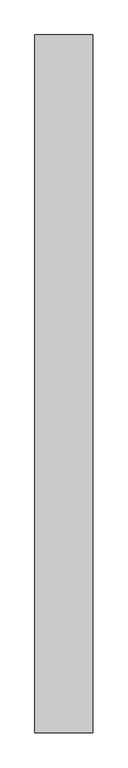
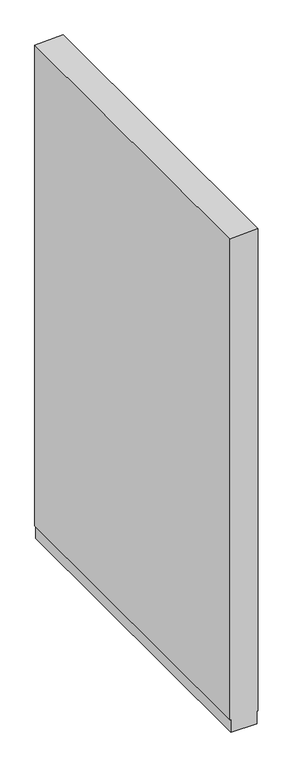
"""IFC4 building model written with IfcOpenShell, lengths in millimetres: proxy geometry, Generic Models 7:Generic Models 1:5:Generic Models 1:5 : Generic Models 7:Generic Models 1:337419:33 : Generic Models 7:Generic Models 1:5:Generic Models 1:5 : Generic Models 7:Generic Models 1:337419:311462."""

from ifc_helpers import new_model, si_unit, frame, origin, place, context, project, spatial, polyline, outline, extrude, source, transform, mapped, element, save


def generic_models_b9c952d6(model_context):
    return source(origin(), model_context, "Body", "SweptSolid", [
        extrude(outline(polyline([(103.1875, 560567.2742239), (3729.5005208, 560567.2742239), (3721.1661458, 560367.2492239), (103.1875, 560367.2492239), (103.1875, 560373.5992239), (7.9375, 560373.5992239), (7.9375, 560560.9242239), (103.1875, 560560.9242239), (103.1875, 560567.2742239)])), frame((0.0, -545590.1663841, 0.0), z_axis=(0.0, 1.0, 0.0), x_axis=(0.0, 0.0, 1.0)), (0.0, 0.0, 1.0), 2406.65),
    ])


if __name__ == "__main__":
    model = new_model("IFC4")
    model_context = context("Model", 3, world=origin())
    ifc_project = project(units=[si_unit("LENGTHUNIT", "METRE", prefix="MILLI")], contexts=[model_context])
    site = spatial("IfcSite", under=ifc_project)
    building = spatial("IfcBuilding", under=site)
    placement = place(None, origin())
    generic_models_shape = generic_models_b9c952d6(model_context)
    element("IfcBuildingElementProxy", 1, Name="Generic Models 7:Generic Models 1:5:Generic Models 1:5 : Generic Models 7:Generic Models 1:337419:33 : Generic Models 7:Generic Models 1:5:Generic Models 1:5 : Generic Models 7:Generic Models 1:337419:311462", ObjectType="Generic Models 7:Generic Models 1:5:Generic Models 1:5 : Generic Models 7:Generic Models 1:337419:33 : Generic Models 7:Generic Models 1:5:Generic Models 1:5 : Generic Models 7:Generic Models 1:337419:311462", at=placement, inside=building, context=model_context, shape_type="MappedRepresentation", body=[
        mapped(generic_models_shape, transform((0.0, 0.0, 0.0), x_axis=(1.0, 0.0, 0.0), y_axis=(0.0, 1.0, 0.0), z_axis=(0.0, 0.0, 1.0))),
    ])
    save(model, "model.ifc")

# Revit data of these elements
# Type "Generic Models 7:Generic Models 1:5:Generic Models 1:5 : Generic Models 7:Generic Models 1:337419:33 : Generic Models 7:Generic Models 1:5:Generic Models 1:5 : Generic Models 7:Generic Models 1:337419:311462"
#   NameOverride = "Generic Models 7:Generic Models 1:5:Generic Models 1:5 : Generic Models 7:Generic Models 1:337419:311462"
#   ObjectTypeOverride = "Generic Models 1:5 : Generic Models 7:Generic Models 1:337419"
#   Reference = "Generic Models 1"
#   Tag = "311462"
# Element 1 (IfcBuildingElementProxy, "Generic Models 7:Generic Models 1:5:Generic Models 1:5 : Generic Models 7:Generic Models 1:337419:33 : Generic Models 7:Generic Models 1:5:Generic Models 1:5 : Generic Models 7:Generic Models 1:337419:311462")
#   Materials on its faces: "FULL CAVITY CLASS A FIBERGLASS INSULATION WITH DURABLE VAPOR BARRIER (BLACK) LINER"
# Materials
#   "FULL CAVITY CLASS A FIBERGLASS INSULATION WITH DURABLE VAPOR BARRIER (BLACK) LINER": class "Unassigned", colour RGB 158 92 175, transparency 0, Cost = 0
